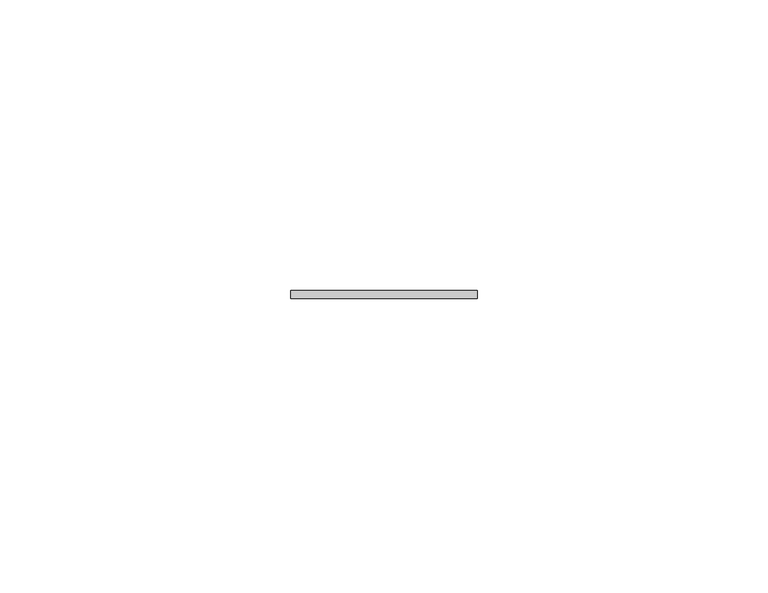
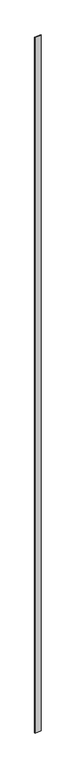
"""IFC4 building model written with IfcOpenShell, lengths in millimetres: proxy geometry, Generic Models 11:Generic Models 1:306267:Generic Models 1:306267 : Generic Models 11:Generic Models 1:306267:300405:Generic Models 1:306267:Generic Models 1:306267 : Generic Models 11:Generic Models 1:306267:300405 : Generic Models 11:Generic Models 1:306267:Generic Models 1:306267 : Generic Models 11:Generic Models 1:306267:300405:24 : Generic Models 11:Generic Models 1:306267:Generic Models 1:306267 : Generic Models 11:Generic Models 1:306267:300405:Generic Models 1:306267:Generic Models 1:306267 : Generic Models 11:Generic Models 1:306267:300405 : Generic Models 11:Generic Models 1:306267:Generic Models 1:306267 : Generic Models 11:Generic Models 1:306267:300405:300182."""

from ifc_helpers import new_model, si_unit, origin, origin_with_axes, place, context, project, spatial, polyline, outline, extrude, source, transform, mapped, element, save


def generic_models_7e357d59(model_context):
    return source(origin(), model_context, "Body", "SweptSolid", [
        extrude(outline(polyline([(596182.8367239, -579027.8802055), (596214.8699389, -579027.8802055), (596214.8699389, -579029.2409731), (596182.8367239, -579029.2409731), (596182.8367239, -579027.8802055)])), origin_with_axes(), (0.0, 0.0, 1.0), 3689.35),
    ])


if __name__ == "__main__":
    model = new_model("IFC4")
    model_context = context("Model", 3, world=origin())
    ifc_project = project(units=[si_unit("LENGTHUNIT", "METRE", prefix="MILLI")], contexts=[model_context])
    site = spatial("IfcSite", under=ifc_project)
    building = spatial("IfcBuilding", under=site)
    placement = place(None, origin())
    generic_models_shape = generic_models_7e357d59(model_context)
    element("IfcBuildingElementProxy", 1, Name="Generic Models 11:Generic Models 1:306267:Generic Models 1:306267 : Generic Models 11:Generic Models 1:306267:300405:Generic Models 1:306267:Generic Models 1:306267 : Generic Models 11:Generic Models 1:306267:300405 : Generic Models 11:Generic Models 1:306267:Generic Models 1:306267 : Generic Models 11:Generic Models 1:306267:300405:24 : Generic Models 11:Generic Models 1:306267:Generic Models 1:306267 : Generic Models 11:Generic Models 1:306267:300405:Generic Models 1:306267:Generic Models 1:306267 : Generic Models 11:Generic Models 1:306267:300405 : Generic Models 11:Generic Models 1:306267:Generic Models 1:306267 : Generic Models 11:Generic Models 1:306267:300405:300182", ObjectType="Generic Models 11:Generic Models 1:306267:Generic Models 1:306267 : Generic Models 11:Generic Models 1:306267:300405:Generic Models 1:306267:Generic Models 1:306267 : Generic Models 11:Generic Models 1:306267:300405 : Generic Models 11:Generic Models 1:306267:Generic Models 1:306267 : Generic Models 11:Generic Models 1:306267:300405:24 : Generic Models 11:Generic Models 1:306267:Generic Models 1:306267 : Generic Models 11:Generic Models 1:306267:300405:Generic Models 1:306267:Generic Models 1:306267 : Generic Models 11:Generic Models 1:306267:300405 : Generic Models 11:Generic Models 1:306267:Generic Models 1:306267 : Generic Models 11:Generic Models 1:306267:300405:300182", at=placement, inside=building, context=model_context, shape_type="MappedRepresentation", body=[
        mapped(generic_models_shape, transform((0.0, 0.0, 0.0), x_axis=(1.0, 0.0, 0.0), y_axis=(0.0, 1.0, 0.0), z_axis=(0.0, 0.0, 1.0))),
    ])
    save(model, "model.ifc")

# Revit data of these elements
# Type "Generic Models 11:Generic Models 1:306267:Generic Models 1:306267 : Generic Models 11:Generic Models 1:306267:300405:Generic Models 1:306267:Generic Models 1:306267 : Generic Models 11:Generic Models 1:306267:300405 : Generic Models 11:Generic Models 1:306267:Generic Models 1:306267 : Generic Models 11:Generic Models 1:306267:300405:24 : Generic Models 11:Generic Models 1:306267:Generic Models 1:306267 : Generic Models 11:Generic Models 1:306267:300405:Generic Models 1:306267:Generic Models 1:306267 : Generic Models 11:Generic Models 1:306267:300405 : Generic Models 11:Generic Models 1:306267:Generic Models 1:306267 : Generic Models 11:Generic Models 1:306267:300405:300182"
#   NameOverride = "Generic Models 11:Generic Models 1:306267:Generic Models 1:306267 : Generic Models 11:Generic Models 1:306267:300405:Generic Models 1:306267:Generic Models 1:306267 : Generic Models 11:Generic Models 1:306267:300405 : Generic Models 11:Generic Models 1:306267:Generic Models 1:306267 : Generic Models 11:Generic Models 1:306267:300405:300182"
#   ObjectTypeOverride = "Generic Models 1:306267:Generic Models 1:306267 : Generic Models 11:Generic Models 1:306267:300405 : Generic Models 11:Generic Models 1:306267:Generic Models 1:306267 : Generic Models 11:Generic Models 1:306267:300405"
#   Reference = "Generic Models 1"
#   Tag = "300182"
# Element 1 (IfcBuildingElementProxy, "Generic Models 11:Generic Models 1:306267:Generic Models 1:306267 : Generic Models 11:Generic Models 1:306267:300405:Generic Models 1:306267:Generic Models 1:306267 : Generic Models 11:Generic Models 1:306267:300405 : Generic Models 11:Generic Models 1:306267:Generic Models 1:306267 : Generic Models 11:Generic Models 1:306267:300405:24 : Generic Models 11:Generic Models 1:306267:Generic Models 1:306267 : Generic Models 11:Generic Models 1:306267:300405:Generic Models 1:306267:Generic Models 1:306267 : Generic Models 11:Generic Models 1:306267:300405 : Generic Models 11:Generic Models 1:306267:Generic Models 1:306267 : Generic Models 11:Generic Models 1:306267:300405:300182")
#   Materials on its faces: "UV STABLE WATER RESISTANT VAPOR PERMEABLE AIR BARRIER (WRB) - WRAP JAMBS/HEADERS - BLACK COLOR"
# Materials
#   "UV STABLE WATER RESISTANT VAPOR PERMEABLE AIR BARRIER (WRB) - WRAP JAMBS/HEADERS - BLACK COLOR": class "Generic", colour RGB 51 162 45, transparency 0, Description = "Polyethylene film membrane", Cost = 0
